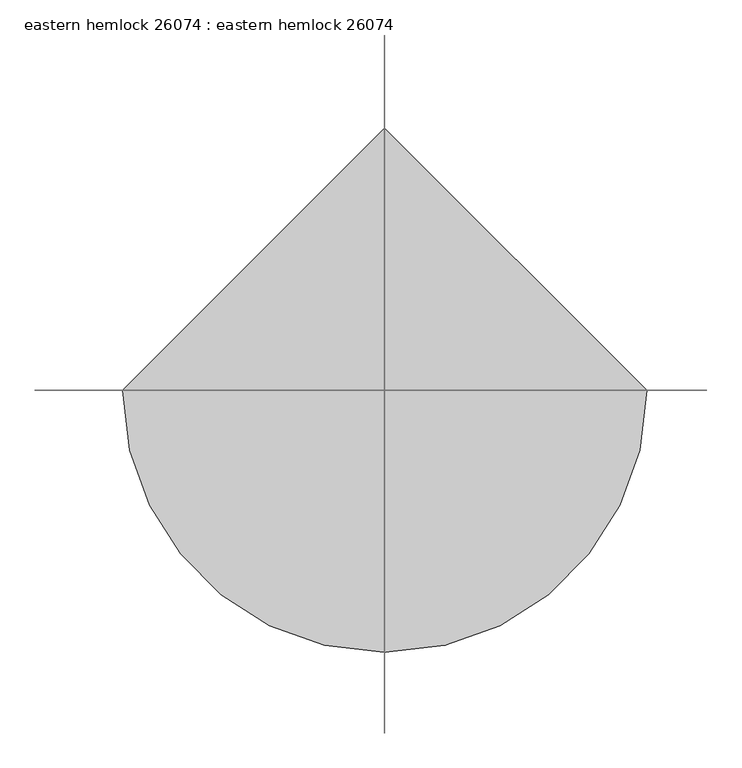
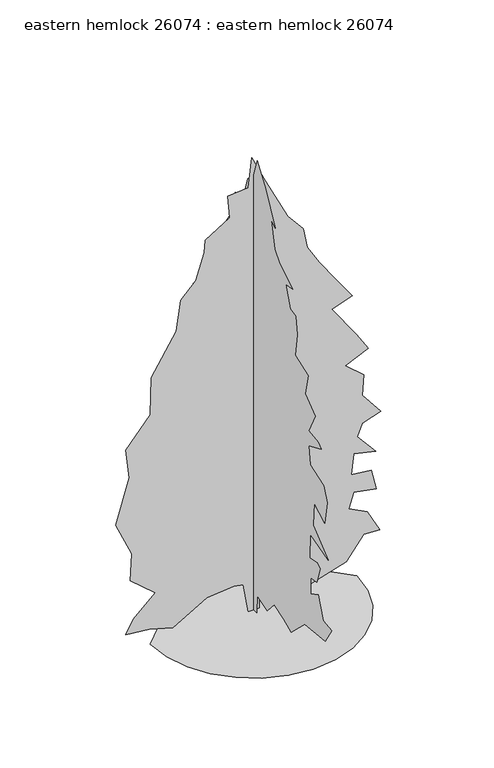
"""IFC4 building model written with IfcOpenShell, lengths in millimetres: proxy geometry, eastern hemlock 26074 : eastern hemlock 26074."""

from ifc_helpers import new_model, si_unit, origin, place, context, project, spatial, triangles, source, transform, mapped, element, save


def eastern_hemlock_26074_eastern_hemlock_26074_32de6804(model_context):
    return source(origin(), model_context, "Body", "Tessellation", [
        triangles([(-1644.9506115, 0.0, 4.68e-05), (-1601.463295, -376.9127495, 4.68e-05), (-1477.6130058, -723.0483805, 4.68e-05), (-1283.3159992, -1028.488167, 4.68e-05), (-1028.488167, -1283.3159992, 4.68e-05), (-723.0483805, -1477.6130058, 4.68e-05), (-376.9127495, -1601.463295, 4.68e-05), (7.19e-05, -1644.9506115, 4.68e-05), (376.9127495, -1601.463295, 4.68e-05), (723.0483805, -1477.6130058, 4.68e-05), (1028.488167, -1283.3159992, 4.68e-05), (1283.3159992, -1028.488167, 4.68e-05), (1477.6130058, -723.0483805, 4.68e-05), (1601.463295, -376.9127495, 4.68e-05), (1644.9506115, 0.0001438, 4.68e-05), (-0.0002157, 1644.9506115, 4.68e-05), (-87.3035192, 3.8e-06, 7.6e-06), (-167.9385319, -2.15e-05, 483.8085503), (-315.7699336, -1.66e-05, 510.6868152), (-749.7665897, 5e-06, 466.2597304), (-1289.7701111, 4.76e-05, 146.9891475), (-1659.6825611, 5.73e-05, 255.3434076), (-2035.9781971, 7.14e-05, 295.6607868), (-1915.0259869, 5.33e-05, 510.6868152), (-1565.6086521, 1.88e-05, 833.2258123), (-1968.782444, 1.56e-05, 1182.6431471), (-1941.9042881, -1.2e-05, 1626.1367889), (-2197.2477139, -3.45e-05, 2190.5800976), (-1982.2215946, -8.72e-05, 2916.2981552), (-2035.9781971, -0.0001137, 3400.0912994), (-1646.2434105, -0.0001579, 3857.0369545), (-1632.8044052, -0.0001954, 4475.2216049), (-1229.6306133, -0.0002514, 5120.3049042), (-1162.4349329, -0.000284, 5617.5600174), (-920.5306578, -0.000309, 5859.4690887), (-786.1393696, -0.0003405, 6289.516095), (-772.700219, -0.0003531, 6491.1159988), (-384.3981211, -0.0003848, 6737.4195694), (-409.8438426, -0.0004058, 7109.3003586), (-87.3032649, -0.0004215, 7136.1737183), (-33.5482861, -0.0004527, 7619.9924423), (181.4795114, -0.0004349, 7163.0720764), (544.3366871, -0.0004075, 6437.344281), (786.2409622, -0.0004004, 6141.6884903), (853.4366426, -0.0003834, 5805.6973709), (1041.584388, -0.0003724, 5483.1688019), (1296.9278137, -0.0003619, 5120.3049042), (1565.7102448, -0.0003512, 4744.0040359), (1243.1712112, -0.0003299, 4623.0747894), (1632.9059978, -0.0003141, 4072.0476677), (1821.0536705, -0.0003039, 3762.9554878), (1458.1973305, -0.0002784, 3601.6909126), (1753.8580627, -0.0002761, 3346.3451614), (1726.9797615, -0.0002549, 3010.3796219), (2022.6406391, -0.0002454, 2634.0790443), (1726.9797615, -0.0002269, 2539.9975777), (1646.3450031, -0.0002113, 2338.4106091), (1942.0058807, -0.0002034, 1988.9932743), (1592.588546, -0.000193, 2069.6280327), (1552.2712395, -0.0001712, 1733.6498486), (1874.810273, -0.0001829, 1693.332542), (1955.4450314, -0.0001664, 1357.3517418), (1592.588546, -0.0001545, 1424.5473495), (1511.9537876, -0.0001358, 1169.2039965), (1807.6145199, -0.0001399, 1021.3736303), (2009.2014885, -0.0001263, 645.078067), (1753.8580627, -0.0001159, 658.5172176), (1471.6364811, -8.19e-05, 295.6607868), (907.1930998, -4.69e-05, 120.9521376), (463.7019287, -3.71e-05, 282.2216543), (87.4051209, -3.35e-05, 497.2477009), (87.4051209, -3.8e-06, 0.0), (4.1e-06, 91.4188294, 5.35e-05), (1.91e-05, 158.6147188, 403.1737919), (3.27e-05, 427.3977493, 456.9302854), (3.49e-05, 548.3498869, 349.4172984), (5.38e-05, 1032.1584372, 255.3434076), (6.46e-05, 1327.8192421, 174.7089036), (8.3e-05, 1730.993034, 188.1480178), (0.0001034, 2026.6537663, 430.0520568), (0.0001188, 2228.2407349, 645.078067), (0.0001026, 1865.3842495, 645.078067), (9.88e-05, 1583.1626678, 940.738872), (0.0001188, 1905.7017014, 1128.8891607), (0.0001321, 2120.7276752, 1249.8412983), (0.0001246, 1784.7494911, 1505.184724), (0.0001421, 1986.3364597, 1787.4063057), (0.0001369, 1798.1886417, 1894.9193653), (0.0001617, 2040.0929169, 2365.288765), (0.0001663, 2053.5345383, 2499.6799805), (0.0001615, 1892.2625507, 2580.3073265), (0.0001691, 1757.8713352, 3037.2526909), (0.0001843, 1865.3842495, 3386.6549103), (0.0001869, 1798.1886417, 3574.8178436), (0.0001943, 1730.993034, 3924.2197723), (0.0001899, 1435.3323017, 4219.9008522), (0.0002082, 1663.7974262, 4488.6835739), (0.0001969, 1260.6236343, 4717.1309669), (0.0002059, 1300.9409409, 4959.040329), (0.0002051, 1085.914967, 5254.6961197), (0.0002166, 1072.4758163, 5657.8697662), (0.0002054, 787.5744564, 5711.8955383), (0.0002156, 790.254162, 6047.6070236), (0.0002156, 494.5933934, 6491.1159988), (0.000223, 508.0325077, 6719.5631012), (0.000215, 293.0064793, 6773.334819), (0.0002206, 158.6142101, 7163.0720764), (0.0002182, -2.6552119, 7324.3366516), (0.0002228, -96.7291975, 7619.9924423), (0.0002019, -338.6349987, 7284.0013229), (0.0001757, -593.9783881, 6786.7717896), (0.0001825, -486.4654012, 6853.9543167), (0.0001655, -580.5392738, 6423.9073105), (0.0001557, -701.4914114, 6276.0797058), (0.0001321, -1077.7869747, 6047.6070236), (0.0001397, -889.6391567, 6020.7336639), (0.0001242, -1010.5912943, 5684.7681244), (0.0001164, -1158.4217331, 5644.4333771), (0.0001062, -1198.7391123, 5362.2139755), (9.69e-05, -1151.8202465, 4980.5791306), (7.72e-05, -1507.8390678, 4851.5221825), (7.04e-05, -1427.2043095, 4502.1199631), (5.19e-05, -1695.9867405, 4287.0839607), (4.93e-05, -1521.2780731, 3937.6564522), (3.67e-05, -1776.6214989, 3897.3467033), (3.11e-05, -1857.2562572, 3830.1638855), (4.17e-05, -1521.2780731, 3682.3359901), (3.11e-05, -1561.595525, 3386.6549103), (1.07e-05, -1937.8910156, 3265.7000839), (-3e-07, -2031.9649246, 3037.2526909), (-8.9e-06, -1964.7693169, 2647.5154335), (9e-06, -1667.4727833, 2801.7696808), (-1.3e-06, -1642.2276672, 2419.0453674), (-3e-05, -2058.8432259, 2083.0671833), (-3.7e-06, -1561.595525, 2217.4583988), (-1.51e-05, -1548.1563744, 1814.2846069), (-2.29e-05, -1749.743343, 1854.6020588), (-2.82e-05, -1830.3781013, 1800.8454563), (-3.24e-05, -1736.3041924, 1518.6238747), (-2.6e-05, -1575.0346756, 1491.7455734), (-3.4e-05, -1575.0346756, 1222.9629971), (-3.98e-05, -1776.6214989, 1330.4760567), (-5.68e-05, -1924.451865, 981.0562511), (-6.78e-05, -2152.9171349, 954.1779499), (-6.84e-05, -1978.2084675, 671.9562956), (-4.48e-05, -1413.7651588, 618.1998384), (-3.88e-05, -1037.4695955, 255.3434076), (-2.7e-05, -835.8826996, 349.4172984), (-1.25e-05, -567.1001595, 430.0520568), (-1.05e-05, -378.9523779, 215.0262827), (4.5e-06, -96.7289432, 295.6607868), (-3.7e-06, -83.2898198, 4.83e-05)], [[15, 16, 1], [14, 15, 1], [14, 1, 2], [13, 14, 2], [13, 2, 3], [13, 3, 4], [12, 13, 4], [11, 12, 4], [11, 4, 5], [11, 5, 6], [11, 6, 7], [11, 7, 8], [11, 8, 9], [11, 9, 10], [40, 41, 42], [57, 58, 59], [65, 66, 67], [61, 62, 63], [60, 61, 63], [22, 23, 24], [54, 55, 56], [47, 48, 49], [50, 51, 52], [22, 24, 25], [71, 72, 17], [71, 17, 18], [38, 39, 40], [21, 22, 25], [20, 21, 25], [64, 65, 67], [40, 42, 43], [38, 40, 43], [64, 67, 68], [64, 68, 69], [64, 69, 70], [64, 70, 71], [49, 50, 52], [36, 37, 38], [36, 38, 43], [35, 36, 43], [35, 43, 44], [35, 44, 45], [35, 45, 46], [34, 35, 46], [33, 34, 46], [33, 46, 47], [33, 47, 49], [32, 33, 49], [31, 32, 49], [31, 49, 52], [30, 31, 52], [29, 30, 52], [28, 29, 52], [27, 28, 52], [27, 52, 53], [27, 53, 54], [27, 54, 56], [27, 56, 57], [27, 57, 59], [27, 59, 60], [26, 27, 60], [25, 26, 60], [20, 25, 60], [19, 20, 60], [18, 19, 60], [71, 18, 60], [64, 71, 60], [64, 60, 63], [133, 134, 135], [110, 111, 112], [114, 115, 116], [80, 81, 82], [108, 109, 110], [125, 126, 127], [124, 125, 127], [143, 144, 145], [84, 85, 86], [130, 131, 132], [96, 97, 98], [86, 87, 88], [141, 142, 143], [143, 145, 146], [141, 143, 146], [79, 80, 82], [151, 152, 73], [151, 73, 74], [120, 121, 122], [129, 130, 132], [128, 129, 132], [104, 105, 106], [122, 123, 124], [83, 84, 86], [100, 101, 102], [137, 138, 139], [136, 137, 139], [136, 139, 140], [78, 79, 82], [78, 82, 83], [77, 78, 83], [89, 90, 91], [146, 147, 148], [117, 118, 119], [149, 150, 151], [108, 110, 112], [107, 108, 112], [106, 107, 112], [106, 112, 113], [104, 106, 113], [76, 77, 83], [75, 76, 83], [88, 89, 91], [103, 104, 113], [102, 103, 113], [102, 113, 114], [102, 114, 116], [102, 116, 117], [102, 117, 119], [102, 119, 120], [100, 102, 120], [99, 100, 120], [98, 99, 120], [98, 120, 122], [98, 122, 124], [96, 98, 124], [96, 124, 127], [96, 127, 128], [96, 128, 132], [95, 96, 132], [94, 95, 132], [93, 94, 132], [92, 93, 132], [92, 132, 133], [92, 133, 135], [91, 92, 135], [88, 91, 135], [88, 135, 136], [86, 88, 136], [83, 86, 136], [75, 83, 136], [74, 75, 136], [74, 136, 140], [151, 74, 140], [149, 151, 140], [149, 140, 141], [149, 141, 146], [149, 146, 148]], closed=False),
    ])


if __name__ == "__main__":
    model = new_model("IFC4")
    model_context = context("Model", 3, world=origin())
    ifc_project = project(units=[si_unit("LENGTHUNIT", "METRE", prefix="MILLI")], contexts=[model_context])
    site = spatial("IfcSite", under=ifc_project)
    building = spatial("IfcBuilding", under=site)
    placement = place(None, origin())
    eastern_hemlock_26074_eastern_hemlock_26074_shape = eastern_hemlock_26074_eastern_hemlock_26074_32de6804(model_context)
    element("IfcBuildingElementProxy", 1, Name="eastern hemlock 26074 : eastern hemlock 26074", ObjectType="eastern hemlock 26074 : eastern hemlock 26074", at=placement, inside=building, context=model_context, shape_type="MappedRepresentation", body=[
        mapped(eastern_hemlock_26074_eastern_hemlock_26074_shape, transform((0.0, 0.0, 0.0), x_axis=(1.0, 0.0, 0.0), y_axis=(0.0, 1.0, 0.0), z_axis=(0.0, 0.0, 1.0))),
    ])
    save(model, "model.ifc")

# Revit data of these elements
# Type "eastern hemlock 26074 : eastern hemlock 26074"
#   built-in parameter 1005195 = "RPC-16-G0VH-QEXX-MT47-S000-ST1L-LVER-AU"
#   Height = 0
